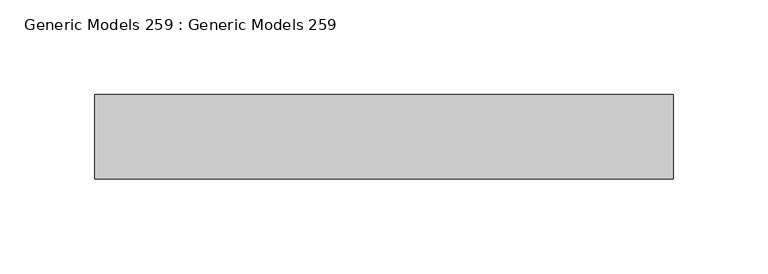
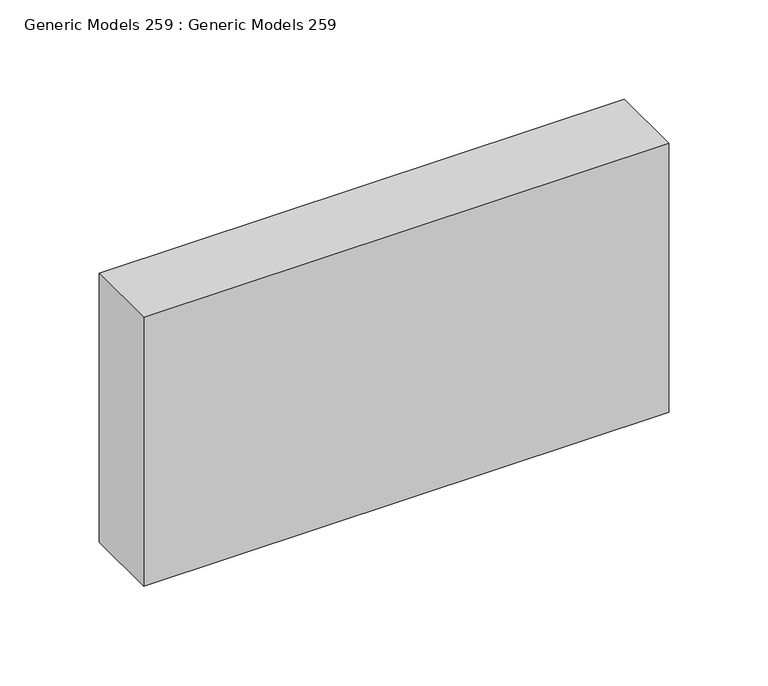
"""IFC4 building model written with IfcOpenShell, lengths in millimetres: proxy geometry, Generic Models 259 : Generic Models 259."""

from ifc_helpers import new_model, si_unit, frame, origin, place, context, project, spatial, polyline, outline, extrude, source, transform, mapped, element, save


def generic_models_259_generic_models_259_25609ed8(model_context):
    return source(origin(), model_context, "Body", "SweptSolid", [
        extrude(outline(polyline([(1389.5910488, 11378.6269662), (1389.5910488, 11334.1769662), (1084.7910488, 11334.1769662), (1084.7910488, 11378.6269662), (1389.5910488, 11378.6269662)])), frame((0.0, 0.0, 126590.552), z_axis=(0.0, 0.0, 1.0), x_axis=(1.0, 0.0, 0.0)), (0.0, 0.0, 1.0), 165.1),
    ])


if __name__ == "__main__":
    model = new_model("IFC4")
    model_context = context("Model", 3, world=origin())
    ifc_project = project(units=[si_unit("LENGTHUNIT", "METRE", prefix="MILLI")], contexts=[model_context])
    site = spatial("IfcSite", under=ifc_project)
    building = spatial("IfcBuilding", under=site)
    placement = place(None, origin())
    generic_models_259_generic_models_259_shape = generic_models_259_generic_models_259_25609ed8(model_context)
    element("IfcBuildingElementProxy", 1, Name="Generic Models 259 : Generic Models 259", ObjectType="Generic Models 259 : Generic Models 259", at=placement, inside=building, context=model_context, shape_type="MappedRepresentation", body=[
        mapped(generic_models_259_generic_models_259_shape, transform((0.0, 0.0, 0.0), x_axis=(1.0, 0.0, 0.0), y_axis=(0.0, 1.0, 0.0), z_axis=(0.0, 0.0, 1.0))),
    ])
    save(model, "model.ifc")

# Revit data of these elements
# Element 1 (IfcBuildingElementProxy, "Generic Models 259 : Generic Models 259")
#   Materials on its faces: "_BLOCKING AS REQUIRED"
# Materials
#   "_BLOCKING AS REQUIRED": class "Generic", colour RGB 177 130 114, transparency 0, Cost = 0
